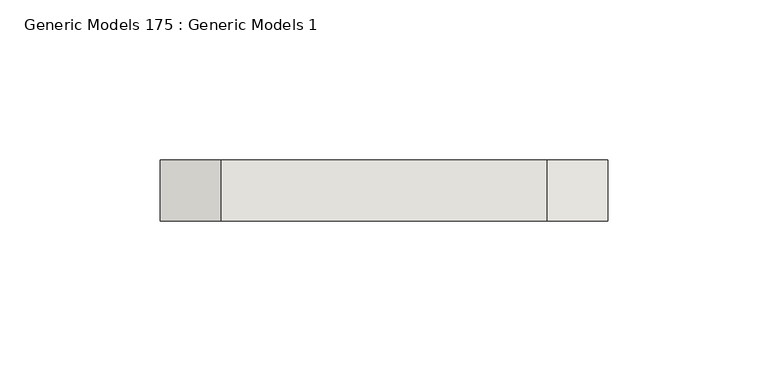
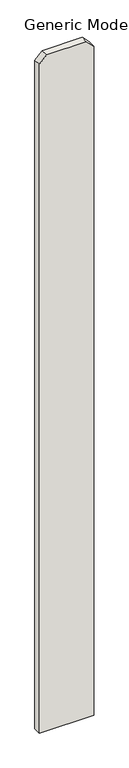
"""IFC4 building model written with IfcOpenShell, lengths in millimetres: wall geometry, Generic Models 175 : Generic Models 1."""

from ifc_helpers import new_model, si_unit, frame, origin, place, context, project, spatial, polyline, outline, extrude, source, transform, mapped, element, save


def generic_models_175_generic_models_1_5439058d(model_context):
    return source(origin(), model_context, "Body", "SweptSolid", [
        extrude(outline(polyline([(76.2, 325651.8125), (1885.95, 325651.8125), (1905.0, 325632.7625), (1905.0, 325531.1625), (1885.95, 325512.1125), (76.2, 325512.1125), (76.2, 325651.8125)])), frame((0.0, 547.6875, 0.0), z_axis=(0.0, 1.0, 0.0), x_axis=(0.0, 0.0, 1.0)), (0.0, 0.0, 1.0), 19.05),
    ])


if __name__ == "__main__":
    model = new_model("IFC4")
    model_context = context("Model", 3, world=origin())
    ifc_project = project(units=[si_unit("LENGTHUNIT", "METRE", prefix="MILLI")], contexts=[model_context])
    site = spatial("IfcSite", under=ifc_project)
    building = spatial("IfcBuilding", under=site)
    placement = place(None, origin())
    generic_models_175_generic_models_1_shape = generic_models_175_generic_models_1_5439058d(model_context)
    element("IfcWall", 1, ObjectType="Generic Models 175 : Generic Models 1", at=placement, inside=building, context=model_context, shape_type="MappedRepresentation", body=[
        mapped(generic_models_175_generic_models_1_shape, transform((0.0, 0.0, 0.0), x_axis=(1.0, 0.0, 0.0), y_axis=(0.0, 1.0, 0.0), z_axis=(0.0, 0.0, 1.0))),
    ])
    save(model, "model.ifc")

# Revit data of these elements
# Element 1 (IfcWall, "Generic Models 175 : Generic Models 1")
#   Materials on its faces: "VERTICAL 1X6 CEDAR PLANKS W/ CLEAR WOOD SEALER"
# Materials
#   "VERTICAL 1X6 CEDAR PLANKS W/ CLEAR WOOD SEALER": class "Wood", colour RGB 234 198 147, transparency 0, Description = "Pinus Echinata", Cost = 0
